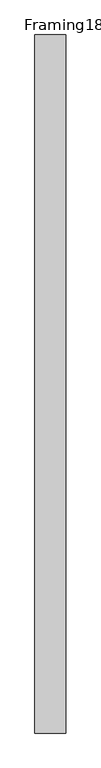
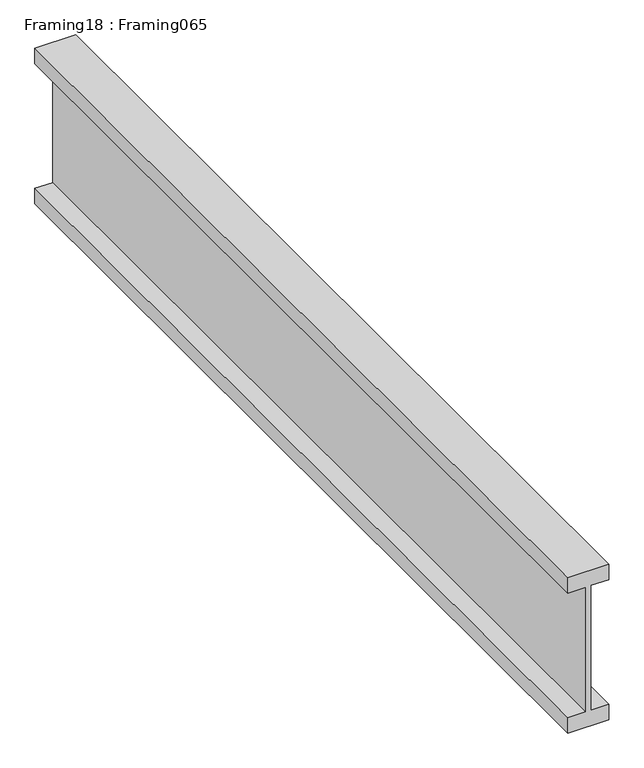
"""IFC4 building model written with IfcOpenShell, lengths in millimetres: proxy geometry, Framing18 : Framing065."""

from ifc_helpers import new_model, si_unit, frame, origin, place, context, project, spatial, polyline, outline, extrude, source, transform, mapped, element, save


def framing18_framing065_252a1c86(model_context):
    return source(origin(), model_context, "Body", "SweptSolid", [
        extrude(outline(polyline([(40077.771, 8096.295938), (39792.021, 8096.295938), (39792.021, 8057.402188), (39757.096, 8057.402188), (39757.096, 8146.302188), (39792.021, 8146.302188), (39792.021, 8107.408438), (40077.771, 8107.408438), (40077.771, 8146.302188), (40112.696, 8146.302188), (40112.696, 8057.402188), (40077.771, 8057.402188), (40077.771, 8096.295938)])), frame((0.0, -3747.9491938, 0.0), z_axis=(0.0, 1.0, 0.0), x_axis=(0.0, 0.0, 1.0)), (0.0, 0.0, 1.0), 2000.0),
    ])


if __name__ == "__main__":
    model = new_model("IFC4")
    model_context = context("Model", 3, world=origin())
    ifc_project = project(units=[si_unit("LENGTHUNIT", "METRE", prefix="MILLI")], contexts=[model_context])
    site = spatial("IfcSite", under=ifc_project)
    building = spatial("IfcBuilding", under=site)
    placement = place(None, origin())
    framing18_framing065_shape = framing18_framing065_252a1c86(model_context)
    element("IfcBuildingElementProxy", 1, Name="Framing18 : Framing065", ObjectType="Framing18 : Framing065", at=placement, inside=building, context=model_context, shape_type="MappedRepresentation", body=[
        mapped(framing18_framing065_shape, transform((0.0, 0.0, 0.0), x_axis=(1.0, 0.0, 0.0), y_axis=(0.0, 1.0, 0.0), z_axis=(0.0, 0.0, 1.0))),
    ])
    save(model, "model.ifc")

# Revit data of these elements
# Type "Framing18 : Framing065"
#   NameOverride = "Framing065"
# Element 1 (IfcBuildingElementProxy, "Framing18 : Framing065")
#   Materials on its faces: "WOOD FRAMING (SEE STRUCT DWGS)"
# Materials
#   "WOOD FRAMING (SEE STRUCT DWGS)": class "Unassigned", colour RGB 224 188 168, transparency 0, Cost = 0
